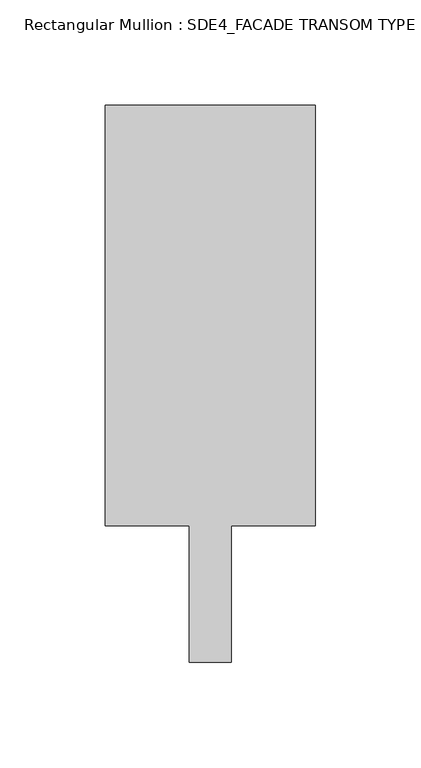
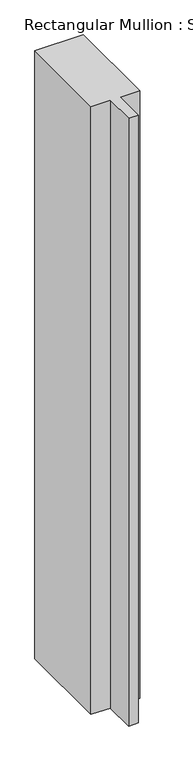
"""IFC4 building model written with IfcOpenShell, lengths in millimetres: member geometry, Rectangular Mullion : SDE4_FACADE TRANSOM TYPE 2."""

from ifc_helpers import new_model, si_unit, frame, origin, place, context, project, spatial, polyline, outline, extrude, source, transform, mapped, element, save


def rectangular_mullion_sde4_facade_transom_type_2_aaaf434f(model_context):
    return source(origin(), model_context, "Body", "SweptSolid", [
        extrude(outline(polyline([(50.0, 132.5), (50.0, -67.5), (10.0, -67.5), (10.0, -132.5), (-10.0, -132.5), (-10.0, -67.5), (-50.0, -67.5), (-50.0, 132.5), (50.0, 132.5)])), frame((0.0, 0.0, -1323.8789692), z_axis=(0.0, 0.0, 1.0), x_axis=(1.0, 0.0, 0.0)), (0.0, 0.0, 1.0), 1323.8789692),
    ])


if __name__ == "__main__":
    model = new_model("IFC4")
    model_context = context("Model", 3, world=origin())
    ifc_project = project(units=[si_unit("LENGTHUNIT", "METRE", prefix="MILLI")], contexts=[model_context])
    site = spatial("IfcSite", under=ifc_project)
    building = spatial("IfcBuilding", under=site)
    placement = place(None, origin())
    rectangular_mullion_sde4_facade_transom_type_2_shape = rectangular_mullion_sde4_facade_transom_type_2_aaaf434f(model_context)
    element("IfcMember", 1, ObjectType="Rectangular Mullion : SDE4_FACADE TRANSOM TYPE 2", at=placement, inside=building, context=model_context, shape_type="MappedRepresentation", body=[
        mapped(rectangular_mullion_sde4_facade_transom_type_2_shape, transform((0.0, 0.0, 0.0), x_axis=(1.0, 0.0, 0.0), y_axis=(0.0, 1.0, 0.0), z_axis=(0.0, 0.0, 1.0))),
    ])
    save(model, "model.ifc")

# Revit data of these elements
# Type "Rectangular Mullion : SDE4_FACADE TRANSOM TYPE 2"
#   built-in parameter 1007322 = 0.869423 (stored number, unit not read)
#   built-in parameter 1007321 = 0.164042 (stored number, unit not read)
#   built-in parameter 1007320 = 0.164042 (stored number, unit not read)
